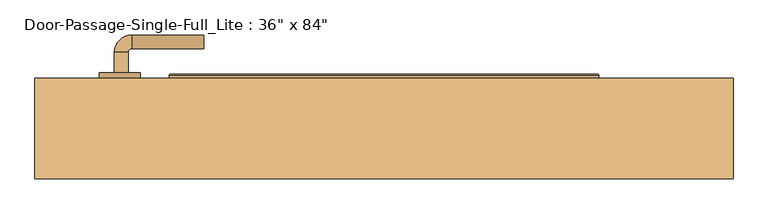
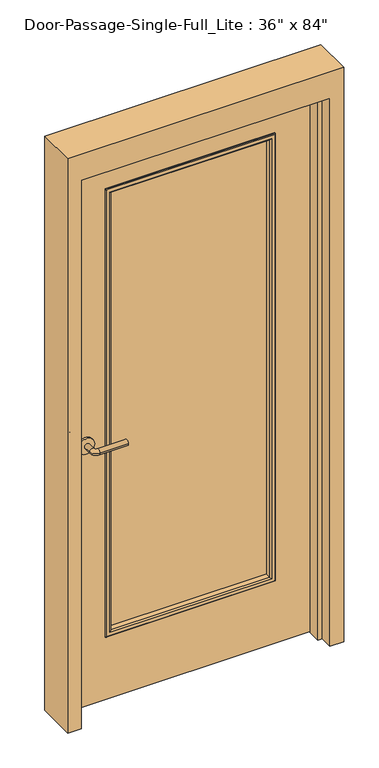
"""IFC4 building model written with IfcOpenShell, lengths in millimetres: door geometry."""

from ifc_helpers import new_model, si_unit, point, frame, frame_2d, origin, place, context, project, spatial, polyline, circle_curve, ellipse_curve, trimmed, segment, composite_curve, outline, extrude, faceted_brep, source, transform, mapped, element, save
from ifc_brep_helpers import plane_surface, cylinder_surface, revolved_surface, advanced_brep


def door_e8956f10(model_context):
    return source(origin(), model_context, "Body", "SolidModel", [
        advanced_brep(
        [(-392.190625, -9.5875, 1016.0), (-372.190625, -9.5875, 1016.0), (-372.190625, -39.5875, 1016.0), (-392.190625, -39.5875, 1016.0), (-367.190625, -44.5875, 1016.0), (-367.190625, -64.5875, 1016.0), (-262.190625, -64.5875, 1016.0), (-262.190625, -44.5875, 1016.0)],
        [
            (0, 1, circle_curve(frame((-382.190625, -9.5875, 1016.0), z_axis=(0.0, 1.0, 0.0), x_axis=(1.0, 0.0, 0.0)), 10.0)),
            (1, 0, circle_curve(frame((-382.190625, -9.5875, 1016.0), z_axis=(0.0, 1.0, 0.0), x_axis=(1.0, 0.0, 0.0)), 10.0)),
            (1, 2),
            (2, 3, circle_curve(frame((-382.190625, -39.5875, 1016.0), z_axis=(0.0, 1.0, 0.0), x_axis=(1.0, 0.0, 0.0)), 10.0)),
            (3, 0),
            (3, 2, circle_curve(frame((-382.190625, -39.5875, 1016.0), z_axis=(0.0, 1.0, 0.0), x_axis=(1.0, 0.0, 0.0)), 10.0)),
            (4, 5, circle_curve(frame((-367.190625, -54.5875, 1016.0), z_axis=(-1.0, 0.0, 0.0), x_axis=(0.0, 1.0, 0.0)), 10.0)),
            (5, 3, circle_curve(frame((-367.190625, -39.5875, 1016.0), z_axis=(0.0, 0.0, -1.0), x_axis=(-1.0, 0.0, 0.0)), 25.0)),
            (2, 4, circle_curve(frame((-367.190625, -39.5875, 1016.0), z_axis=(0.0, 0.0, 1.0), x_axis=(-1.0, 0.0, 0.0)), 5.0)),
            (5, 4, circle_curve(frame((-367.190625, -54.5875, 1016.0), z_axis=(-1.0, 0.0, 0.0), x_axis=(0.0, 1.0, 0.0)), 10.0)),
            (6, 7, circle_curve(frame((-262.190625, -54.5875, 1016.0), z_axis=(1.0, 0.0, 0.0), x_axis=(0.0, 1.0, 0.0)), 10.0)),
            (7, 6, circle_curve(frame((-262.190625, -54.5875, 1016.0), z_axis=(1.0, 0.0, 0.0), x_axis=(0.0, 1.0, 0.0)), 10.0)),
            (4, 7),
            (6, 5),
        ],
        [
            plane_surface(frame((-382.190625, -9.5875, 1016.0), z_axis=(0.0, 1.0, 0.0), x_axis=(0.0, 0.0, 1.0))),
            cylinder_surface(frame((-382.190625, -9.5875, 1016.0), z_axis=(0.0, 1.0, 0.0), x_axis=(1.0, 0.0, 0.0)), 10.0),
            revolved_surface(trimmed(ellipse_curve(frame((-382.190625, -39.5875, 1016.0), z_axis=(0.0, -1.0, 0.0), x_axis=(1.0, 0.0, 0.0)), 10.0, 10.0), [point((-392.190625, -39.5875, 1016.0))], [point((-372.190625, -39.5875, 1016.0))], True, "CARTESIAN"), (-367.190625, -39.5875, 1016.0), (0.0, 0.0, -1.0)),
            revolved_surface(trimmed(ellipse_curve(frame((-382.190625, -39.5875, 1016.0), z_axis=(0.0, -1.0, 0.0), x_axis=(1.0, 0.0, 0.0)), 10.0, 10.0), [point((-372.190625, -39.5875, 1016.0))], [point((-392.190625, -39.5875, 1016.0))], True, "CARTESIAN"), (-367.190625, -39.5875, 1016.0), (0.0, 0.0, -1.0)),
            plane_surface(frame((-262.190625, -54.5875, 1016.0), z_axis=(1.0, 0.0, 0.0), x_axis=(0.0, 0.0, 1.0))),
            cylinder_surface(frame((-367.190625, -54.5875, 1016.0), z_axis=(-1.0, 0.0, 0.0), x_axis=(0.0, 1.0, 0.0)), 10.0),
        ],
        [
            (0, [[1, 2]]),
            (1, [[3, 4, 5, -2]]),
            (1, [[-5, 6, -3, -1]]),
            (2, [[7, 8, -4, 9]]),
            (3, [[10, -9, -6, -8]]),
            (4, [[11, 12]]),
            (5, [[13, -11, 14, -7]]),
            (5, [[-14, -12, -13, -10]]),
        ],
    ),
        extrude(outline(composite_curve([segment(trimmed(circle_curve(frame_2d((1016.0, -384.690625)), 30.0), [point((1016.0, -414.690625))], [point((1016.0, -354.690625))], False, "CARTESIAN"), True, "CONTINUOUS"), segment(trimmed(circle_curve(frame_2d((1016.0, -384.690625)), 30.0), [point((1016.0, -354.690625))], [point((1016.0, -414.690625))], False, "CARTESIAN"), True, "CONTINUOUS")], self_intersect=False)), frame((0.0, -9.5875, 0.0), z_axis=(0.0, 1.0, 0.0), x_axis=(0.0, 0.0, 1.0)), (0.0, 0.0, 1.0), 8.0),
        advanced_brep(
        [(-392.190625, 50.8625, 1016.0), (-372.190625, 50.8625, 1016.0), (-392.190625, 80.8625, 1016.0), (-372.190625, 80.8625, 1016.0), (-367.190625, 85.8625, 1016.0), (-367.190625, 105.8625, 1016.0), (-262.190625, 105.8625, 1016.0), (-262.190625, 85.8625, 1016.0)],
        [
            (0, 1, circle_curve(frame((-382.190625, 50.8625, 1016.0), z_axis=(0.0, -1.0, 0.0), x_axis=(1.0, 0.0, 0.0)), 10.0)),
            (1, 0, circle_curve(frame((-382.190625, 50.8625, 1016.0), z_axis=(0.0, -1.0, 0.0), x_axis=(1.0, 0.0, 0.0)), 10.0)),
            (0, 2),
            (2, 3, circle_curve(frame((-382.190625, 80.8625, 1016.0), z_axis=(0.0, -1.0, 0.0), x_axis=(1.0, 0.0, 0.0)), 10.0)),
            (3, 1),
            (3, 2, circle_curve(frame((-382.190625, 80.8625, 1016.0), z_axis=(0.0, -1.0, 0.0), x_axis=(1.0, 0.0, 0.0)), 10.0)),
            (4, 3, circle_curve(frame((-367.190625, 80.8625, 1016.0), z_axis=(0.0, 0.0, 1.0), x_axis=(-1.0, 0.0, 0.0)), 5.0)),
            (2, 5, circle_curve(frame((-367.190625, 80.8625, 1016.0), z_axis=(0.0, 0.0, -1.0), x_axis=(-1.0, 0.0, 0.0)), 25.0)),
            (5, 4, circle_curve(frame((-367.190625, 95.8625, 1016.0), z_axis=(-1.0, 0.0, 0.0), x_axis=(0.0, -1.0, 0.0)), 10.0)),
            (4, 5, circle_curve(frame((-367.190625, 95.8625, 1016.0), z_axis=(-1.0, 0.0, 0.0), x_axis=(0.0, -1.0, 0.0)), 10.0)),
            (6, 7, circle_curve(frame((-262.190625, 95.8625, 1016.0), z_axis=(1.0, 0.0, 0.0), x_axis=(0.0, -1.0, 0.0)), 10.0)),
            (7, 6, circle_curve(frame((-262.190625, 95.8625, 1016.0), z_axis=(1.0, 0.0, 0.0), x_axis=(0.0, -1.0, 0.0)), 10.0)),
            (5, 6),
            (7, 4),
        ],
        [
            plane_surface(frame((-382.190625, 50.8625, 1016.0), z_axis=(0.0, -1.0, 0.0), x_axis=(0.0, 0.0, 1.0))),
            cylinder_surface(frame((-382.190625, 50.8625, 1016.0), z_axis=(0.0, -1.0, 0.0), x_axis=(1.0, 0.0, 0.0)), 10.0),
            revolved_surface(trimmed(ellipse_curve(frame((-382.190625, 80.8625, 1016.0), z_axis=(0.0, -1.0, 0.0), x_axis=(1.0, 0.0, 0.0)), 10.0, 10.0), [point((-392.190625, 80.8625, 1016.0))], [point((-372.190625, 80.8625, 1016.0))], True, "CARTESIAN"), (-367.190625, 80.8625, 1016.0), (0.0, 0.0, -1.0)),
            revolved_surface(trimmed(ellipse_curve(frame((-382.190625, 80.8625, 1016.0), z_axis=(0.0, -1.0, 0.0), x_axis=(1.0, 0.0, 0.0)), 10.0, 10.0), [point((-372.190625, 80.8625, 1016.0))], [point((-392.190625, 80.8625, 1016.0))], True, "CARTESIAN"), (-367.190625, 80.8625, 1016.0), (0.0, 0.0, -1.0)),
            plane_surface(frame((-262.190625, 95.8625, 1016.0), z_axis=(1.0, 0.0, 0.0), x_axis=(0.0, 0.0, 1.0))),
            cylinder_surface(frame((-367.190625, 95.8625, 1016.0), z_axis=(-1.0, 0.0, 0.0), x_axis=(0.0, -1.0, 0.0)), 10.0),
        ],
        [
            (0, [[1, 2]]),
            (1, [[-1, 3, 4, 5]]),
            (1, [[-2, -5, 6, -3]]),
            (2, [[7, -4, 8, 9]]),
            (3, [[-8, -6, -7, 10]]),
            (4, [[11, 12]]),
            (5, [[-9, 13, -12, 14]]),
            (5, [[-10, -14, -11, -13]]),
        ],
    ),
        extrude(outline(composite_curve([segment(trimmed(circle_curve(frame_2d((1016.0, -384.690625)), 30.0), [point((1016.0, -414.690625))], [point((1016.0, -354.690625))], False, "CARTESIAN"), True, "CONTINUOUS"), segment(trimmed(circle_curve(frame_2d((1016.0, -384.690625)), 30.0), [point((1016.0, -354.690625))], [point((1016.0, -414.690625))], False, "CARTESIAN"), True, "CONTINUOUS")], self_intersect=False)), frame((0.0, 42.8625, 0.0), z_axis=(0.0, 1.0, 0.0), x_axis=(0.0, 0.0, 1.0)), (0.0, 0.0, 1.0), 8.0),
        extrude(outline(polyline([(304.8, 17.4625), (-304.8, 17.4625), (-304.8, 23.8125), (304.8, 23.8125), (304.8, 17.4625)])), frame((0.0, 0.0, 254.0), z_axis=(0.0, 0.0, 1.0), x_axis=(1.0, 0.0, 0.0)), (0.0, 0.0, 1.0), 1727.2),
        faceted_brep([(457.2, -6.35, 0.0), (457.2, 42.8625, 0.0), (508.0, 42.8625, 0.0), (508.0, -103.1875, 0.0), (457.2, -103.1875, 0.0), (457.2, -53.975, 0.0), (441.325, -53.975, 0.0), (441.325, -6.35, 0.0), (457.2, -6.35, 2133.6), (457.2, 42.8625, 2133.6), (-457.2, 42.8625, 2133.6), (-457.2, 42.8625, 0.0), (-508.0, 42.8625, 0.0), (-508.0, 42.8625, 2235.2), (508.0, 42.8625, 2235.2), (508.0, -103.1875, 2235.2), (-508.0, -103.1875, 2235.2), (-508.0, -103.1875, 0.0), (-457.2, -103.1875, 0.0), (-457.2, -103.1875, 2133.6), (457.2, -103.1875, 2133.6), (457.2, -53.975, 2133.6), (-457.2, -53.975, 2133.6), (-457.2, -53.975, 0.0), (-441.325, -53.975, 0.0), (-441.325, -53.975, 2117.725), (441.325, -53.975, 2117.725), (441.325, -6.35, 2117.725), (-441.325, -6.35, 2117.725), (-441.325, -6.35, 0.0), (-457.2, -6.35, 0.0), (-457.2, -6.35, 2133.6)], [[[0, 1, 2, 3, 4, 5, 6, 7]], [[1, 0, 8, 9]], [[2, 1, 9, 10, 11, 12, 13, 14]], [[3, 2, 14, 15]], [[4, 3, 15, 16, 17, 18, 19, 20]], [[5, 4, 20, 21]], [[6, 5, 21, 22, 23, 24, 25, 26]], [[7, 6, 26, 27]], [[0, 7, 27, 28, 29, 30, 31, 8]], [[9, 8, 31, 10]], [[20, 19, 22, 21]], [[26, 25, 28, 27]], [[12, 11, 30, 29, 24, 23, 18, 17]], [[11, 10, 31, 30]], [[13, 12, 17, 16]], [[19, 18, 23, 22]], [[25, 24, 29, 28]], [[15, 14, 13, 16]]]),
        extrude(outline(polyline([(2133.6, -457.2), (0.0, -457.2), (0.0, 457.2), (2133.6, 457.2), (2133.6, -457.2)]), holes=[polyline([(1981.2, -304.8), (1981.2, 304.8), (254.0, 304.8), (254.0, -304.8), (1981.2, -304.8)])]), frame((0.0, -1.5875, 0.0), z_axis=(0.0, 1.0, 0.0), x_axis=(0.0, 0.0, 1.0)), (0.0, 0.0, 1.0), 44.45),
        advanced_brep(
        [(-304.8, 23.8125, 1981.2), (-304.8, 42.8625, 1981.2), (-304.8, 42.8625, 254.0), (-304.8, 23.8125, 254.0), (-292.8, 43.8625, 1969.2), (-292.8, 23.8125, 1969.2), (-292.8, 23.8125, 266.0), (-292.8, 43.8625, 266.0), (-297.8, 48.8625, 1974.2), (-297.8, 48.8625, 261.0), (-312.8, 46.8625, 1989.2), (-310.8, 48.8625, 1987.2), (-310.8, 48.8625, 248.0), (-312.8, 46.8625, 246.0), (-312.8, 42.8625, 1989.2), (-312.8, 42.8625, 246.0), (304.8, 42.8625, 254.0), (304.8, 23.8125, 254.0), (292.8, 23.8125, 266.0), (292.8, 43.8625, 266.0), (297.8, 48.8625, 261.0), (310.8, 48.8625, 248.0), (312.8, 46.8625, 246.0), (312.8, 42.8625, 246.0), (304.8, 42.8625, 1981.2), (304.8, 23.8125, 1981.2), (292.8, 23.8125, 1969.2), (292.8, 43.8625, 1969.2), (297.8, 48.8625, 1974.2), (310.8, 48.8625, 1987.2), (312.8, 46.8625, 1989.2), (312.8, 42.8625, 1989.2)],
        [
            (0, 1),
            (1, 2),
            (2, 3),
            (3, 0),
            (4, 5),
            (5, 6),
            (6, 7),
            (7, 4),
            (8, 4, ellipse_curve(frame((-297.8, 43.8625, 1974.2), z_axis=(-0.7071067811865475, 0.0, -0.7071067811865475), x_axis=(-0.7071067811865474, 0.0, 0.7071067811865476)), 7.0710678, 5.0)),
            (7, 9, ellipse_curve(frame((-297.8, 43.8625, 261.0), z_axis=(-0.7071067811865475, 0.0, 0.7071067811865475), x_axis=(0.7071067811865474, 0.0, 0.7071067811865476)), 7.0710678, 5.0)),
            (9, 8),
            (10, 11, ellipse_curve(frame((-310.8, 46.8625, 1987.2), z_axis=(-0.7071067811865475, 0.0, -0.7071067811865475), x_axis=(-0.7071067811865474, 0.0, 0.7071067811865476)), 2.8284271, 2.0)),
            (11, 12),
            (12, 13, ellipse_curve(frame((-310.8, 46.8625, 248.0), z_axis=(-0.7071067811865475, 0.0, 0.7071067811865475), x_axis=(0.7071067811865474, 0.0, 0.7071067811865476)), 2.8284271, 2.0)),
            (13, 10),
            (14, 10),
            (13, 15),
            (15, 14),
            (2, 16),
            (16, 17),
            (17, 3),
            (6, 18),
            (18, 19),
            (19, 7),
            (19, 20, ellipse_curve(frame((297.8, 43.8625, 261.0), z_axis=(-0.7071067811865475, 0.0, -0.7071067811865475), x_axis=(-0.7071067811865476, 0.0, 0.7071067811865474)), 7.0710678, 5.0)),
            (20, 9),
            (12, 21),
            (21, 22, ellipse_curve(frame((310.8, 46.8625, 248.0), z_axis=(-0.7071067811865475, 0.0, -0.7071067811865475), x_axis=(-0.7071067811865476, 0.0, 0.7071067811865474)), 2.8284271, 2.0)),
            (22, 13),
            (22, 23),
            (23, 15),
            (16, 24),
            (24, 25),
            (25, 17),
            (18, 26),
            (26, 27),
            (27, 19),
            (27, 28, ellipse_curve(frame((297.8, 43.8625, 1974.2), z_axis=(0.7071067811865475, 0.0, -0.7071067811865475), x_axis=(-0.7071067811865474, 0.0, -0.7071067811865476)), 7.0710678, 5.0)),
            (28, 20),
            (21, 29),
            (29, 30, ellipse_curve(frame((310.8, 46.8625, 1987.2), z_axis=(0.7071067811865475, 0.0, -0.7071067811865475), x_axis=(-0.7071067811865474, 0.0, -0.7071067811865476)), 2.8284271, 2.0)),
            (30, 22),
            (30, 31),
            (31, 23),
            (31, 14),
            (1, 24),
            (0, 25),
            (5, 26),
            (4, 27),
            (8, 28),
            (11, 29),
            (10, 30),
        ],
        [
            plane_surface(frame((-304.8, 42.8625, 1981.2), z_axis=(-1.0, 0.0, 0.0), x_axis=(0.0, 0.0, -1.0))),
            plane_surface(frame((-292.8, 23.8125, 1969.2), z_axis=(1.0, 0.0, 0.0), x_axis=(0.0, 0.0, -1.0))),
            cylinder_surface(frame((-297.8, 43.8625, 1981.2), z_axis=(0.0, 0.0, 1.0), x_axis=(-1.0, 0.0, 0.0)), 5.0),
            cylinder_surface(frame((-310.8, 46.8625, 1981.2), z_axis=(0.0, 0.0, 1.0), x_axis=(-1.0, 0.0, 0.0)), 2.0),
            plane_surface(frame((-312.8, 46.8625, 1989.2), z_axis=(-1.0, 0.0, 0.0), x_axis=(0.0, 0.0, -1.0))),
            plane_surface(frame((-304.8, 42.8625, 254.0), z_axis=(0.0, 0.0, -1.0), x_axis=(1.0, 0.0, 0.0))),
            plane_surface(frame((-292.8, 23.8125, 266.0), z_axis=(0.0, 0.0, 1.0), x_axis=(1.0, 0.0, 0.0))),
            cylinder_surface(frame((-304.8, 43.8625, 261.0), z_axis=(-1.0, 0.0, 0.0), x_axis=(0.0, 0.0, -1.0)), 5.0),
            cylinder_surface(frame((-304.8, 46.8625, 248.0), z_axis=(-1.0, 0.0, 0.0), x_axis=(0.0, 0.0, -1.0)), 2.0),
            plane_surface(frame((-312.8, 46.8625, 246.0), z_axis=(0.0, 0.0, -1.0), x_axis=(1.0, 0.0, 0.0))),
            plane_surface(frame((304.8, 42.8625, 254.0), z_axis=(1.0, 0.0, 0.0), x_axis=(0.0, 0.0, 1.0))),
            plane_surface(frame((292.8, 23.8125, 266.0), z_axis=(-1.0, 0.0, 0.0), x_axis=(0.0, 0.0, 1.0))),
            cylinder_surface(frame((297.8, 43.8625, 254.0), z_axis=(0.0, 0.0, -1.0), x_axis=(1.0, 0.0, 0.0)), 5.0),
            cylinder_surface(frame((310.8, 46.8625, 254.0), z_axis=(0.0, 0.0, -1.0), x_axis=(1.0, 0.0, 0.0)), 2.0),
            plane_surface(frame((312.8, 46.8625, 246.0), z_axis=(1.0, 0.0, 0.0), x_axis=(0.0, 0.0, 1.0))),
            plane_surface(frame((312.8, 42.8625, 1989.2), z_axis=(0.0, -1.0, 0.0), x_axis=(-1.0, 0.0, 0.0))),
            plane_surface(frame((304.8, 42.8625, 1981.2), z_axis=(0.0, 0.0, 1.0), x_axis=(-1.0, 0.0, 0.0))),
            plane_surface(frame((304.8, 23.8125, 1981.2), z_axis=(0.0, -1.0, 0.0), x_axis=(-1.0, 0.0, 0.0))),
            plane_surface(frame((292.8, 23.8125, 1969.2), z_axis=(0.0, 0.0, -1.0), x_axis=(-1.0, 0.0, 0.0))),
            cylinder_surface(frame((304.8, 43.8625, 1974.2), z_axis=(1.0, 0.0, 0.0), x_axis=(0.0, 0.0, 1.0)), 5.0),
            plane_surface(frame((297.8, 48.8625, 1974.2), z_axis=(0.0, 1.0, 0.0), x_axis=(-1.0, 0.0, 0.0))),
            cylinder_surface(frame((304.8, 46.8625, 1987.2), z_axis=(1.0, 0.0, 0.0), x_axis=(0.0, 0.0, 1.0)), 2.0),
            plane_surface(frame((312.8, 46.8625, 1989.2), z_axis=(0.0, 0.0, 1.0), x_axis=(-1.0, 0.0, 0.0))),
        ],
        [
            (0, [[1, 2, 3, 4]]),
            (1, [[5, 6, 7, 8]]),
            (2, [[9, -8, 10, 11]]),
            (3, [[12, 13, 14, 15]]),
            (4, [[16, -15, 17, 18]]),
            (5, [[-3, 19, 20, 21]]),
            (6, [[-7, 22, 23, 24]]),
            (7, [[-10, -24, 25, 26]]),
            (8, [[-14, 27, 28, 29]]),
            (9, [[-17, -29, 30, 31]]),
            (10, [[-20, 32, 33, 34]]),
            (11, [[-23, 35, 36, 37]]),
            (12, [[-25, -37, 38, 39]]),
            (13, [[-28, 40, 41, 42]]),
            (14, [[-30, -42, 43, 44]]),
            (15, [[-31, -44, 45, -18], [46, -32, -19, -2]]),
            (16, [[-33, -46, -1, 47]]),
            (17, [[-21, -34, -47, -4], [48, -35, -22, -6]]),
            (18, [[-36, -48, -5, 49]]),
            (19, [[-38, -49, -9, 50]]),
            (20, [[51, -40, -27, -13], [-26, -39, -50, -11]]),
            (21, [[-41, -51, -12, 52]]),
            (22, [[-43, -52, -16, -45]]),
        ],
    ),
        advanced_brep(
        [(-304.8, 17.4625, 254.0), (-304.8, -1.5875, 254.0), (-304.8, -1.5875, 1981.2), (-304.8, 17.4625, 1981.2), (-292.8, -2.5875, 266.0), (-292.8, 17.4625, 266.0), (-292.8, 17.4625, 1969.2), (-292.8, -2.5875, 1969.2), (-297.8, -7.5875, 261.0), (-297.8, -7.5875, 1974.2), (-312.8, -5.5875, 246.0), (-310.8, -7.5875, 248.0), (-310.8, -7.5875, 1987.2), (-312.8, -5.5875, 1989.2), (-312.8, -1.5875, 246.0), (-312.8, -1.5875, 1989.2), (304.8, -1.5875, 1981.2), (304.8, 17.4625, 1981.2), (292.8, 17.4625, 1969.2), (292.8, -2.5875, 1969.2), (297.8, -7.5875, 1974.2), (310.8, -7.5875, 1987.2), (312.8, -5.5875, 1989.2), (312.8, -1.5875, 1989.2), (304.8, -1.5875, 254.0), (304.8, 17.4625, 254.0), (292.8, 17.4625, 266.0), (292.8, -2.5875, 266.0), (297.8, -7.5875, 261.0), (310.8, -7.5875, 248.0), (312.8, -5.5875, 246.0), (312.8, -1.5875, 246.0)],
        [
            (0, 1),
            (1, 2),
            (2, 3),
            (3, 0),
            (4, 5),
            (5, 6),
            (6, 7),
            (7, 4),
            (8, 4, ellipse_curve(frame((-297.8, -2.5875, 261.0), z_axis=(-0.7071067811865475, 0.0, 0.7071067811865475), x_axis=(-0.7071067811865474, 0.0, -0.7071067811865476)), 7.0710678, 5.0)),
            (7, 9, ellipse_curve(frame((-297.8, -2.5875, 1974.2), z_axis=(-0.7071067811865475, 0.0, -0.7071067811865475), x_axis=(0.7071067811865474, 0.0, -0.7071067811865476)), 7.0710678, 5.0)),
            (9, 8),
            (10, 11, ellipse_curve(frame((-310.8, -5.5875, 248.0), z_axis=(-0.7071067811865475, 0.0, 0.7071067811865475), x_axis=(-0.7071067811865474, 0.0, -0.7071067811865476)), 2.8284271, 2.0)),
            (11, 12),
            (12, 13, ellipse_curve(frame((-310.8, -5.5875, 1987.2), z_axis=(-0.7071067811865475, 0.0, -0.7071067811865475), x_axis=(0.7071067811865474, 0.0, -0.7071067811865476)), 2.8284271, 2.0)),
            (13, 10),
            (14, 10),
            (13, 15),
            (15, 14),
            (2, 16),
            (16, 17),
            (17, 3),
            (6, 18),
            (18, 19),
            (19, 7),
            (19, 20, ellipse_curve(frame((297.8, -2.5875, 1974.2), z_axis=(-0.7071067811865475, 0.0, 0.7071067811865475), x_axis=(-0.7071067811865476, 0.0, -0.7071067811865474)), 7.0710678, 5.0)),
            (20, 9),
            (12, 21),
            (21, 22, ellipse_curve(frame((310.8, -5.5875, 1987.2), z_axis=(-0.7071067811865475, 0.0, 0.7071067811865475), x_axis=(-0.7071067811865476, 0.0, -0.7071067811865474)), 2.8284271, 2.0)),
            (22, 13),
            (22, 23),
            (23, 15),
            (16, 24),
            (24, 25),
            (25, 17),
            (18, 26),
            (26, 27),
            (27, 19),
            (27, 28, ellipse_curve(frame((297.8, -2.5875, 261.0), z_axis=(0.7071067811865475, 0.0, 0.7071067811865475), x_axis=(-0.7071067811865474, 0.0, 0.7071067811865476)), 7.0710678, 5.0)),
            (28, 20),
            (21, 29),
            (29, 30, ellipse_curve(frame((310.8, -5.5875, 248.0), z_axis=(0.7071067811865475, 0.0, 0.7071067811865475), x_axis=(-0.7071067811865474, 0.0, 0.7071067811865476)), 2.8284271, 2.0)),
            (30, 22),
            (30, 31),
            (31, 23),
            (31, 14),
            (1, 24),
            (0, 25),
            (5, 26),
            (4, 27),
            (8, 28),
            (11, 29),
            (10, 30),
        ],
        [
            plane_surface(frame((-304.8, -1.5875, 254.0), z_axis=(-1.0, 0.0, 0.0), x_axis=(0.0, 0.0, 1.0))),
            plane_surface(frame((-292.8, 17.4625, 266.0), z_axis=(1.0, 0.0, 0.0), x_axis=(0.0, 0.0, 1.0))),
            cylinder_surface(frame((-297.8, -2.5875, 254.0), z_axis=(0.0, 0.0, -1.0), x_axis=(-1.0, 0.0, 0.0)), 5.0),
            cylinder_surface(frame((-310.8, -5.5875, 254.0), z_axis=(0.0, 0.0, -1.0), x_axis=(-1.0, 0.0, 0.0)), 2.0),
            plane_surface(frame((-312.8, -5.5875, 246.0), z_axis=(-1.0, 0.0, 0.0), x_axis=(0.0, 0.0, 1.0))),
            plane_surface(frame((-304.8, -1.5875, 1981.2), z_axis=(0.0, 0.0, 1.0), x_axis=(1.0, 0.0, 0.0))),
            plane_surface(frame((-292.8, 17.4625, 1969.2), z_axis=(0.0, 0.0, -1.0), x_axis=(1.0, 0.0, 0.0))),
            cylinder_surface(frame((-304.8, -2.5875, 1974.2), z_axis=(-1.0, 0.0, 0.0), x_axis=(0.0, 0.0, 1.0)), 5.0),
            cylinder_surface(frame((-304.8, -5.5875, 1987.2), z_axis=(-1.0, 0.0, 0.0), x_axis=(0.0, 0.0, 1.0)), 2.0),
            plane_surface(frame((-312.8, -5.5875, 1989.2), z_axis=(0.0, 0.0, 1.0), x_axis=(1.0, 0.0, 0.0))),
            plane_surface(frame((304.8, -1.5875, 1981.2), z_axis=(1.0, 0.0, 0.0), x_axis=(0.0, 0.0, -1.0))),
            plane_surface(frame((292.8, 17.4625, 1969.2), z_axis=(-1.0, 0.0, 0.0), x_axis=(0.0, 0.0, -1.0))),
            cylinder_surface(frame((297.8, -2.5875, 1981.2), z_axis=(0.0, 0.0, 1.0), x_axis=(1.0, 0.0, 0.0)), 5.0),
            cylinder_surface(frame((310.8, -5.5875, 1981.2), z_axis=(0.0, 0.0, 1.0), x_axis=(1.0, 0.0, 0.0)), 2.0),
            plane_surface(frame((312.8, -5.5875, 1989.2), z_axis=(1.0, 0.0, 0.0), x_axis=(0.0, 0.0, -1.0))),
            plane_surface(frame((312.8, -1.5875, 246.0), z_axis=(0.0, 1.0, 0.0), x_axis=(-1.0, 0.0, 0.0))),
            plane_surface(frame((304.8, -1.5875, 254.0), z_axis=(0.0, 0.0, -1.0), x_axis=(-1.0, 0.0, 0.0))),
            plane_surface(frame((304.8, 17.4625, 254.0), z_axis=(0.0, 1.0, 0.0), x_axis=(-1.0, 0.0, 0.0))),
            plane_surface(frame((292.8, 17.4625, 266.0), z_axis=(0.0, 0.0, 1.0), x_axis=(-1.0, 0.0, 0.0))),
            cylinder_surface(frame((304.8, -2.5875, 261.0), z_axis=(1.0, 0.0, 0.0), x_axis=(0.0, 0.0, -1.0)), 5.0),
            plane_surface(frame((297.8, -7.5875, 261.0), z_axis=(0.0, -1.0, 0.0), x_axis=(-1.0, 0.0, 0.0))),
            cylinder_surface(frame((304.8, -5.5875, 248.0), z_axis=(1.0, 0.0, 0.0), x_axis=(0.0, 0.0, -1.0)), 2.0),
            plane_surface(frame((312.8, -5.5875, 246.0), z_axis=(0.0, 0.0, -1.0), x_axis=(-1.0, 0.0, 0.0))),
        ],
        [
            (0, [[1, 2, 3, 4]]),
            (1, [[5, 6, 7, 8]]),
            (2, [[9, -8, 10, 11]]),
            (3, [[12, 13, 14, 15]]),
            (4, [[16, -15, 17, 18]]),
            (5, [[-3, 19, 20, 21]]),
            (6, [[-7, 22, 23, 24]]),
            (7, [[-10, -24, 25, 26]]),
            (8, [[-14, 27, 28, 29]]),
            (9, [[-17, -29, 30, 31]]),
            (10, [[-20, 32, 33, 34]]),
            (11, [[-23, 35, 36, 37]]),
            (12, [[-25, -37, 38, 39]]),
            (13, [[-28, 40, 41, 42]]),
            (14, [[-30, -42, 43, 44]]),
            (15, [[-31, -44, 45, -18], [46, -32, -19, -2]]),
            (16, [[-33, -46, -1, 47]]),
            (17, [[-21, -34, -47, -4], [48, -35, -22, -6]]),
            (18, [[-36, -48, -5, 49]]),
            (19, [[-38, -49, -9, 50]]),
            (20, [[51, -40, -27, -13], [-26, -39, -50, -11]]),
            (21, [[-41, -51, -12, 52]]),
            (22, [[-43, -52, -16, -45]]),
        ],
    ),
    ])


if __name__ == "__main__":
    model = new_model("IFC4")
    model_context = context("Model", 3, world=origin())
    ifc_project = project(units=[si_unit("LENGTHUNIT", "METRE", prefix="MILLI")], contexts=[model_context])
    site = spatial("IfcSite", under=ifc_project)
    building = spatial("IfcBuilding", under=site)
    placement = place(None, origin())
    door_shape = door_e8956f10(model_context)
    element("IfcDoor", 1, ObjectType="Door-Passage-Single-Full_Lite : 36\" x 84\"", at=placement, inside=building, context=model_context, shape_type="MappedRepresentation", body=[
        mapped(door_shape, transform((0.0, 0.0, 0.0), x_axis=(1.0, 0.0, 0.0), y_axis=(0.0, 1.0, 0.0), z_axis=(0.0, 0.0, 1.0))),
    ])
    save(model, "model.ifc")

# Revit data of these elements
# Type "Door-Passage-Single-Full_Lite : 36\" x 84\""
#   Type Mark = "52"
#   Assembly Code = "B2030100"
#   Analytic Construction = "Wooden"
#   Thickness = 0' - 1 3/4"
#   Thermal Resistance (R) = 2.5876 (h·ft²·°F)/BTU
#   Swing Angle [instance default] = 90.00°
#   Strike Height = 3' - 4"
#   Rough Width [instance default] = 3' - 4"
#   Rough Height [instance default] = 7' - 4"
#   MF Opening Height [instance default] = 0' - 4"
#   MF Opening Width [instance default] = 0' - 4"
#   Inset Calculate [instance default] = 0' - 4"
#   Masonry Inset [instance default] = 0' - 1"
#   Height = 7' - 0"
#   Width = 3' - 0"
#   Heat Transfer Coefficient (U) = 0.3865 BTU/(h·ft²·°F)
#   Masonry Frame Depth = 0' - 5 3/4"
#   Masonry Frame [instance default] = yes
#   Function = 1
#   Dry Wall Frame [instance default] = no
#   Panel Material = Wood - Birch
#   Glazing = Glass
#   Glass Stop Material = Metal - Paint Finish - Grey
#   Frame Material = Metal - Paint Finish - Grey
#   Door Handle Material = Aluminum
#   Visual Light Transmittance = 0
#   Solar Heat Gain Coefficient = 0
#   Wall Closure = (empty or 0)
# Element 1 (IfcDoor, "Door-Passage-Single-Full_Lite : 36\" x 84\"")
#   Materials on its faces: "Metal - Paint Finish - Grey", "Aluminum", "Wood - Birch", "Glass"
# Materials
#   "Wood - Birch": class "Wood", colour RGB 166 116 52, transparency 0, Cost = 0
#   "Glass": class "Glass", colour RGB 0 128 192, transparency 0.75, Description = "Soda Lime Glass", Cost = 0
#   "Metal - Paint Finish - Grey": class "Paint", colour RGB 104 104 104, transparency 0, Cost = 0
#   "Aluminum": class "Metal", colour RGB 247 247 247, transparency 0, Description = "Aluminum 6061", Cost = 0
